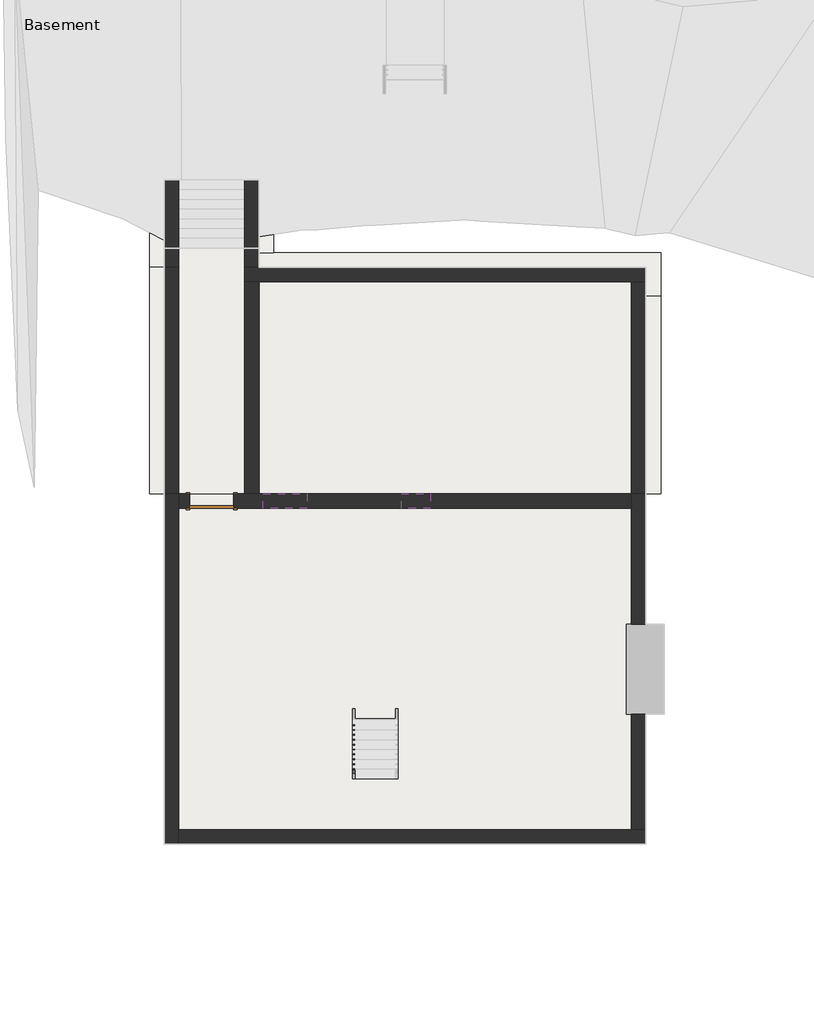
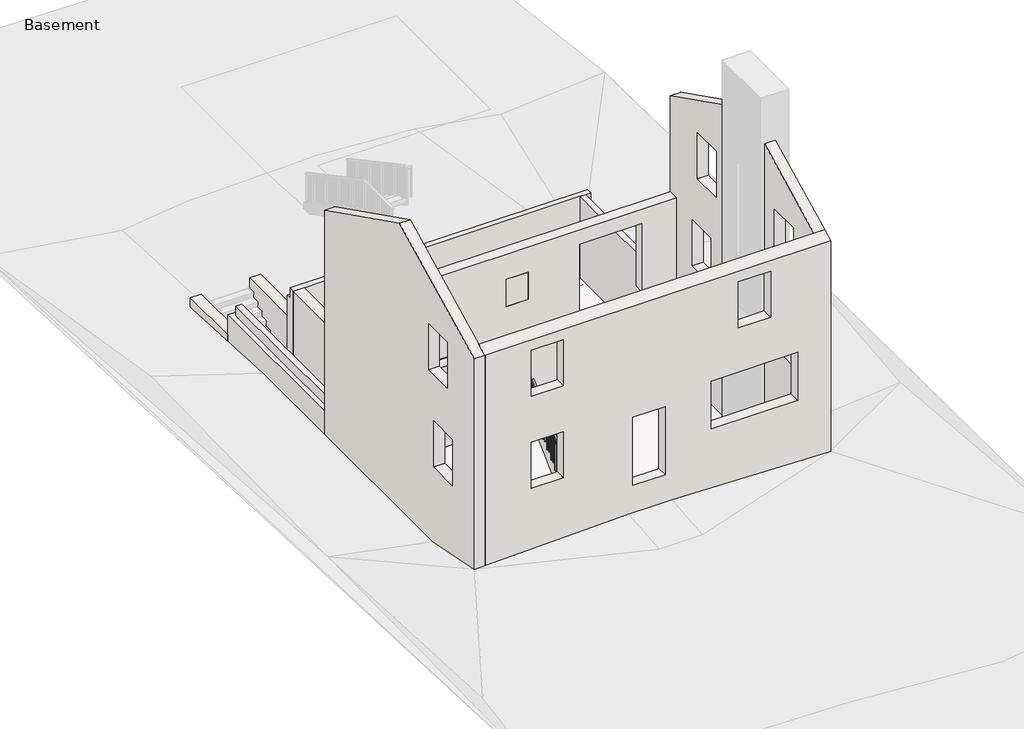
# One storey, part 1 of 3: 13 walls, 6 footings, 4 slabs, 1 door, 1 railing.
"""IFC4 building model written with IfcOpenShell, lengths in millimetres."""

import ifcopenshell
import ifcopenshell.guid

model = None  # the IFC model being written
_history = None  # IfcOwnerHistory: only IFC2X3 demands one
_inside = {}  # id of a spatial element -> (the spatial element, [elements in it])
_under = {}  # id of a project, library or spatial element -> (it, [spatial elements below it])
_declared = {}  # id of a project -> (the project, [libraries it declares])
_typed = {}  # id of a type object -> (the type object, [elements of that type])
_made_of = {}  # id of a material, layer set ... -> (it, [elements and type objects made of it])


def new_model(schema):
    """Start an empty IFC model of exactly this schema.

    Asked for "IFC4X3", IfcOpenShell would pick the latest addendum, in which some entities
    have other attributes; the version numbers below select the first issue.
    IFC2X3 requires an IfcOwnerHistory on every rooted entity: one is made here for all.
    """
    global model, _history
    if schema == "IFC4X3":
        model = ifcopenshell.file(schema_version=(4, 3, 0, 0))
    else:
        model = ifcopenshell.file(schema=schema)
    _inside.clear()
    _under.clear()
    _declared.clear()
    _typed.clear()
    _made_of.clear()
    _history = None
    if model.schema == "IFC2X3":
        org = make("IfcOrganization", Name="unknown")
        user = make(
            "IfcPersonAndOrganization",
            ThePerson=make("IfcPerson", FamilyName="unknown"),
            TheOrganization=org,
        )
        app = make(
            "IfcApplication",
            ApplicationDeveloper=org,
            Version="unknown",
            ApplicationFullName="unknown",
            ApplicationIdentifier="unknown",
        )
        _history = make(
            "IfcOwnerHistory",
            OwningUser=user,
            OwningApplication=app,
            ChangeAction="ADDED",
            CreationDate=0,
        )
    return model


def make(cls, **values):
    """One entity of the class cls with the attributes given. An attribute that is None is left unset."""
    return model.create_entity(
        cls, **{name: value for name, value in values.items() if value is not None}
    )


def rooted(cls, **values):
    """An entity with a GlobalId (a new one), such as an element, a storey or a relation."""
    return make(cls, GlobalId=ifcopenshell.guid.new(), OwnerHistory=_history, **values)


def si_unit(unit_type, name, prefix=None):
    """IfcSIUnit, for example si_unit("LENGTHUNIT", "METRE", prefix="MILLI")."""
    return make("IfcSIUnit", UnitType=unit_type, Prefix=prefix, Name=name)


def assignment(units):
    """IfcUnitAssignment: the units of a project."""
    return None if units is None else make("IfcUnitAssignment", Units=units)


def point(xyz):
    """IfcCartesianPoint."""
    return None if xyz is None else make("IfcCartesianPoint", Coordinates=xyz)


def direction(xyz):
    """IfcDirection."""
    return None if xyz is None else make("IfcDirection", DirectionRatios=xyz)


def frame(location, z_axis=None, x_axis=None):
    """IfcAxis2Placement3D, a coordinate frame: its origin and axes. An axis left out is left unset."""
    return make(
        "IfcAxis2Placement3D",
        Location=point(location),
        Axis=direction(z_axis),
        RefDirection=direction(x_axis),
    )


def origin():
    """The frame at (0, 0, 0) with its axes left unset."""
    return frame((0.0, 0.0, 0.0))


def origin_with_axes():
    """The frame at (0, 0, 0) with the z axis (0, 0, 1) and the x axis (1, 0, 0) written out."""
    return frame((0.0, 0.0, 0.0), z_axis=(0.0, 0.0, 1.0), x_axis=(1.0, 0.0, 0.0))


def place(relative_to, where):
    """IfcLocalPlacement: puts the frame where relative to a parent placement (None: the world)."""
    return make(
        "IfcLocalPlacement", PlacementRelTo=relative_to, RelativePlacement=where
    )


def context(
    kind, dimensions, precision=None, world=None, true_north=None, identifier=None
):
    """IfcGeometricRepresentationContext, for example the 3D "Model" context."""
    return make(
        "IfcGeometricRepresentationContext",
        ContextIdentifier=identifier,
        ContextType=kind,
        CoordinateSpaceDimension=dimensions,
        Precision=precision,
        WorldCoordinateSystem=world,
        TrueNorth=true_north,
    )


def project(units=None, contexts=None):
    """IfcProject with its units and contexts."""
    return rooted(
        "IfcProject",
        Name="project",
        RepresentationContexts=contexts,
        UnitsInContext=assignment(units),
    )


def spatial(cls, under=None, at=None, **own):
    """A site, building, storey or space (cls), placed at a placement, below another one or the project."""
    s = rooted(cls, ObjectPlacement=at, **own)
    if under is not None:
        _under.setdefault(under.id(), (under, []))[1].append(s)
    return s


def polyline(points):
    """IfcPolyline through the points."""
    return make("IfcPolyline", Points=[point(p) for p in points])


def outline(outer, holes=None, kind="AREA"):
    """IfcArbitraryClosedProfileDef: a profile drawn as a closed curve; with holes, ...WithVoids."""
    if holes is None:
        return make("IfcArbitraryClosedProfileDef", ProfileType=kind, OuterCurve=outer)
    return make(
        "IfcArbitraryProfileDefWithVoids",
        ProfileType=kind,
        OuterCurve=outer,
        InnerCurves=holes,
    )


def extrude(swept, where, along, depth):
    """IfcExtrudedAreaSolid: the profile swept, set in the frame where, extruded along a direction by depth."""
    return make(
        "IfcExtrudedAreaSolid",
        SweptArea=swept,
        Position=where,
        ExtrudedDirection=direction(along),
        Depth=depth,
    )


def faces_of(points, faces, orient=None, outer=None):
    """IfcFace entities. A face is a list of loops; a loop is a list of indices into points, from 0.

    orient and outer hold one flag for each loop. By default every Orientation is true, the
    first loop of a face is its IfcFaceOuterBound and the others are IfcFaceBound.
    """
    made = []
    for i, loops in enumerate(faces):
        bounds = []
        for j, loop in enumerate(loops):
            is_outer = j == 0 if outer is None else outer[i][j]
            bounds.append(
                make(
                    "IfcFaceOuterBound" if is_outer else "IfcFaceBound",
                    Bound=make("IfcPolyLoop", Polygon=[points[k] for k in loop]),
                    Orientation=True if orient is None else orient[i][j],
                )
            )
        made.append(make("IfcFace", Bounds=bounds))
    return made


def faceted_brep(points, faces, orient=None, outer=None, voids=None):
    """IfcFacetedBrep: a solid bounded by flat faces; with voids (closed shells), ...WithVoids."""
    shared = [point(p) for p in points]
    hull = make("IfcClosedShell", CfsFaces=faces_of(shared, faces, orient, outer))
    if voids is None:
        return make("IfcFacetedBrep", Outer=hull)
    return make(
        "IfcFacetedBrepWithVoids",
        Outer=hull,
        Voids=[
            make(cls, CfsFaces=faces_of(shared, fs, o, b)) for cls, fs, o, b in voids
        ],
    )


def shape(context_of_items, identifier, shape_type, items):
    """IfcShapeRepresentation: the items that make up one representation, for example the "Body"."""
    return make(
        "IfcShapeRepresentation",
        ContextOfItems=context_of_items,
        RepresentationIdentifier=identifier,
        RepresentationType=shape_type,
        Items=items,
    )


def source(mapping_origin, context_of_items, identifier, shape_type, items):
    """IfcRepresentationMap: a shape defined once, which mapped items show again and again."""
    return make(
        "IfcRepresentationMap",
        MappingOrigin=mapping_origin,
        MappedRepresentation=shape(context_of_items, identifier, shape_type, items),
    )


def transform(
    local_origin,
    x_axis=None,
    y_axis=None,
    z_axis=None,
    scale=None,
    scale2=None,
    scale3=None,
    uniform=True,
):
    """IfcCartesianTransformationOperator3D, or its non-uniform kind. x_axis, y_axis, z_axis: its Axis1, 2, 3."""
    if uniform:
        return make(
            "IfcCartesianTransformationOperator3D",
            Axis1=direction(x_axis),
            Axis2=direction(y_axis),
            LocalOrigin=point(local_origin),
            Scale=scale,
            Axis3=direction(z_axis),
        )
    return make(
        "IfcCartesianTransformationOperator3DnonUniform",
        Axis1=direction(x_axis),
        Axis2=direction(y_axis),
        LocalOrigin=point(local_origin),
        Scale=scale,
        Axis3=direction(z_axis),
        Scale2=scale2,
        Scale3=scale3,
    )


def mapped(mapping_source, mapping_target):
    """IfcMappedItem: shows the shape of a source again, moved by a transform."""
    return make(
        "IfcMappedItem", MappingSource=mapping_source, MappingTarget=mapping_target
    )


def made_of(thing, what):
    """Note that an element or type object is made of a material, layer set ...; save() writes the relation."""
    if what is not None:
        _made_of.setdefault(what.id(), (what, []))[1].append(thing)
    return thing


def element(
    cls,
    number,
    at=None,
    inside=None,
    cuts=None,
    type_object=None,
    material=None,
    context=None,
    identifier="Body",
    shape_type=None,
    held_by="IfcProductDefinitionShape",
    body=None,
    shapes=None,
    **own,
):
    """One element of the class cls, such as IfcWall. Its Tag is "e" and its number.

    at: its placement. inside: the storey or other place that contains it. cuts: it is an
    opening in that element (IfcRelVoidsElement). A single representation is given by context,
    identifier, shape_type and body (its items); several are given by shapes. held_by: the class
    of the entity that holds the representations. save() writes the other relations.
    """
    e = rooted(cls, Tag="e%d" % number, ObjectPlacement=at, **own)
    if body is not None:
        shapes = [shape(context, identifier, shape_type, body)]
    if shapes is not None:
        e.Representation = make(held_by, Representations=shapes)
    if inside is not None:
        _inside.setdefault(inside.id(), (inside, []))[1].append(e)
    if cuts is not None:
        rooted(
            "IfcRelVoidsElement", RelatingBuildingElement=cuts, RelatedOpeningElement=e
        )
    if type_object is not None:
        _typed.setdefault(type_object.id(), (type_object, []))[1].append(e)
    return made_of(e, material)


def aggregate(whole, parts):
    """IfcRelAggregates: a whole, such as a stair, and the parts it consists of."""
    return rooted("IfcRelAggregates", RelatingObject=whole, RelatedObjects=parts)


def save(model, path):
    """Write the relations noted so far, then the file.

    IfcRelAggregates (storeys below a building ...), IfcRelContainedInSpatialStructure (elements
    in a storey), IfcRelDefinesByType, IfcRelAssociatesMaterial and IfcRelDeclares: one each for
    every whole, place, type object, material and project.
    """
    for whole, parts in _under.values():
        aggregate(whole, parts)
    for where, things in _inside.values():
        rooted(
            "IfcRelContainedInSpatialStructure",
            RelatedElements=things,
            RelatingStructure=where,
        )
    for kind, things in _typed.values():
        rooted("IfcRelDefinesByType", RelatedObjects=things, RelatingType=kind)
    for what, things in _made_of.values():
        rooted("IfcRelAssociatesMaterial", RelatedObjects=things, RelatingMaterial=what)
    for by, libraries in _declared.values():
        rooted("IfcRelDeclares", RelatingContext=by, RelatedDefinitions=libraries)
    model.write(path)


def door_03272193(model_context):
    return source(origin(), model_context, "Body", "SweptSolid", [
        extrude(outline(polyline([(2209.8, -533.4), (0.0, -533.4), (0.0, -457.2), (2133.6, -457.2), (2133.6, 457.2), (0.0, 457.2), (0.0, 533.4), (2209.8, 533.4), (2209.8, -533.4)])), frame((0.0, 152.4, 0.0), z_axis=(0.0, 1.0, 0.0), x_axis=(0.0, 0.0, 1.0)), (0.0, 0.0, 1.0), 25.4),
        extrude(outline(polyline([(2209.8, 533.4), (2209.8, -533.4), (0.0, -533.4), (0.0, -457.2), (2133.6, -457.2), (2133.6, 457.2), (0.0, 457.2), (0.0, 533.4), (2209.8, 533.4)])), frame((0.0, -177.8, 0.0), z_axis=(0.0, 1.0, 0.0), x_axis=(0.0, 0.0, 1.0)), (0.0, 0.0, 1.0), 25.4),
        extrude(outline(polyline([(457.2, 101.6), (-457.2, 101.6), (-457.2, 152.4), (457.2, 152.4), (457.2, 101.6)])), origin_with_axes(), (0.0, 0.0, 1.0), 2133.6),
    ])


model = new_model("IFC4")

# Units and contexts
model_context = context("Model", 3, world=origin())
ifc_project = project(units=[si_unit("LENGTHUNIT", "METRE", prefix="MILLI")], contexts=[model_context])

# Site, building, storey
site = spatial("IfcSite", under=ifc_project)
building = spatial("IfcBuilding", under=site)
storey = spatial("IfcBuildingStorey", under=building, Name="Basement", Elevation=-2667.0)

# Door
placement = place(None, origin())
door_shape = door_03272193(model_context)
element("IfcDoor", 1, ObjectType="Single-Flush : 36\" x 84\"", at=placement, inside=storey, context=model_context, shape_type="MappedRepresentation", body=[
    mapped(door_shape, transform((-4998.5803068, 2999.6888758, -2667.0), x_axis=(-1.0, 0.0, 0.0), y_axis=(0.0, -1.0, 0.0), z_axis=(0.0, 0.0, 1.0))),
])

# Footings
element("IfcFooting", 2, ObjectType="Bearing Footing - 36\" x 12\"", at=placement, inside=storey, context=model_context, shape_type="SweptSolid", body=[
    extrude(outline(polyline([(-5379.5803068, 3152.0888758), (-6293.9803068, 3152.0888758), (-6293.9803068, 7876.4888758), (-5379.5803068, 7876.4888758), (-5379.5803068, 3152.0888758)])), frame((0.0, 0.0, -3073.4), z_axis=(0.0, 0.0, 1.0), x_axis=(1.0, 0.0, 0.0)), (0.0, 0.0, 1.0), 304.8),
])
element("IfcFooting", 3, ObjectType="Bearing Footing - 36\" x 12\"", at=placement, inside=storey, context=model_context, shape_type="Brep", body=[
    faceted_brep([(-4160.3803068, 7266.8888758, -2768.6), (-3703.1803068, 7266.8888758, -2768.6), (3459.6196932, 7266.8888758, -2768.6), (4374.0196932, 7266.8888758, -2768.6), (4374.0196932, 8181.2888758, -2768.6), (-3703.1803068, 8181.2888758, -2768.6), (-4160.3803068, 8181.2888758, -2768.6), (-4160.3803068, 7876.4888758, -2768.6), (-4160.3803068, 7724.0888758, -2768.6), (-4160.3803068, 7571.6888758, -2768.6), (-4160.3803068, 8181.2888758, -3073.4), (4374.0196932, 8181.2888758, -3073.4), (-3703.1803068, 8181.2888758, -3073.4), (-4160.3803068, 7266.8888758, -3073.4), (-4160.3803068, 7571.6888758, -3073.4), (-4160.3803068, 7724.0888758, -3073.4), (-4160.3803068, 7876.4888758, -3073.4), (4374.0196932, 7266.8888758, -3073.4), (3459.6196932, 7266.8888758, -3073.4), (-3703.1803068, 7266.8888758, -3073.4)], [[[0, 1, 2, 3, 4, 5, 6, 7, 8, 9]], [[10, 6, 5, 4, 11, 12]], [[13, 14, 15, 16, 10, 12, 11, 17, 18, 19]], [[0, 13, 19, 18, 17, 3, 2, 1]], [[4, 3, 17, 11]], [[0, 9, 8, 15, 14, 13]], [[8, 7, 6, 10, 16, 15]]]),
])
element("IfcFooting", 4, ObjectType="Bearing Footing - 36\" x 12\"", at=placement, inside=storey, context=model_context, shape_type="SweptSolid", body=[
    extrude(outline(polyline([(4374.0196932, 3152.0888758), (3459.6196932, 3152.0888758), (3459.6196932, 7266.8888758), (4374.0196932, 7266.8888758), (4374.0196932, 3152.0888758)])), frame((0.0, 0.0, -3073.4), z_axis=(0.0, 0.0, 1.0), x_axis=(1.0, 0.0, 0.0)), (0.0, 0.0, 1.0), 304.8),
])
element("IfcFooting", 5, ObjectType="Bearing Footing - 36\" x 12\"", at=placement, inside=storey, context=model_context, shape_type="SweptSolid", body=[
    extrude(outline(polyline([(-3703.1803068, 3152.0888758), (-4617.5803068, 3152.0888758), (-4617.5803068, 7571.6888758), (-4160.3803068, 7571.6888758), (-4160.3803068, 7266.8888758), (-3703.1803068, 7266.8888758), (-3703.1803068, 3152.0888758)])), frame((0.0, 0.0, -3073.4), z_axis=(0.0, 0.0, 1.0), x_axis=(1.0, 0.0, 0.0)), (0.0, 0.0, 1.0), 304.8),
])
element("IfcFooting", 6, ObjectType="Bearing Footing - 36\" x 12\"", at=placement, inside=storey, context=model_context, shape_type="SweptSolid", body=[
    extrude(outline(polyline([(-4617.5803068, 9705.2888758), (-3703.1803068, 9705.2888758), (-3703.1803068, 8181.2888758), (-4160.3803068, 8181.2888758), (-4160.3803068, 7876.4888758), (-4617.5803068, 7876.4888758), (-4617.5803068, 9705.2888758)])), frame((0.0, 0.0, -3073.4), z_axis=(0.0, 0.0, 1.0), x_axis=(1.0, 0.0, 0.0)), (0.0, 0.0, 1.0), 304.8),
])
element("IfcFooting", 7, ObjectType="Bearing Footing - 36\" x 12\"", at=placement, inside=storey, context=model_context, shape_type="SweptSolid", body=[
    extrude(outline(polyline([(-5379.5803068, 7876.4888758), (-6293.9803068, 7876.4888758), (-6293.9803068, 9705.2888758), (-5379.5803068, 9705.2888758), (-5379.5803068, 7876.4888758)])), frame((0.0, 0.0, -3073.4), z_axis=(0.0, 0.0, 1.0), x_axis=(1.0, 0.0, 0.0)), (0.0, 0.0, 1.0), 304.8),
])

# Railing
element("IfcRailing", 8, ObjectType="Handrail - Rectangular", at=placement, inside=storey, context=model_context, shape_type="SweptSolid", body=[
    extrude(outline(polyline([(-2791.5111242, -1631.7331862), (-2791.5111242, -1562.1), (-149.9111242, 914.4), (-149.9111242, 844.7668138), (-2791.5111242, -1631.7331862)])), frame((-2052.1803068, 0.0, 0.0), z_axis=(1.0, 0.0, 0.0), x_axis=(0.0, 1.0, 0.0)), (0.0, 0.0, 1.0), 50.8),
    extrude(outline(polyline([(-241.9861242, 758.4465013), (-241.9861242, -190.5), (-261.0361242, -190.5), (-261.0361242, 740.5871263), (-241.9861242, 758.4465013)])), frame((-2036.3053068, 0.0, 0.0), z_axis=(1.0, 0.0, 0.0), x_axis=(0.0, 1.0, 0.0)), (0.0, 0.0, 1.0), 19.05),
    extrude(outline(polyline([(-343.5861242, 663.1965013), (-343.5861242, -190.5), (-362.6361242, -190.5), (-362.6361242, 645.3371263), (-343.5861242, 663.1965013)])), frame((-2036.3053068, 0.0, 0.0), z_axis=(1.0, 0.0, 0.0), x_axis=(0.0, 1.0, 0.0)), (0.0, 0.0, 1.0), 19.05),
    extrude(outline(polyline([(-445.1861242, 567.9465013), (-445.1861242, -381.0), (-464.2361242, -381.0), (-464.2361242, 550.0871263), (-445.1861242, 567.9465013)])), frame((-2036.3053068, 0.0, 0.0), z_axis=(1.0, 0.0, 0.0), x_axis=(0.0, 1.0, 0.0)), (0.0, 0.0, 1.0), 19.05),
    extrude(outline(polyline([(-546.7861242, 472.6965013), (-546.7861242, -381.0), (-565.8361242, -381.0), (-565.8361242, 454.8371263), (-546.7861242, 472.6965013)])), frame((-2036.3053068, 0.0, 0.0), z_axis=(1.0, 0.0, 0.0), x_axis=(0.0, 1.0, 0.0)), (0.0, 0.0, 1.0), 19.05),
    extrude(outline(polyline([(-648.3861242, 377.4465013), (-648.3861242, -571.5), (-667.4361242, -571.5), (-667.4361242, 359.5871263), (-648.3861242, 377.4465013)])), frame((-2036.3053068, 0.0, 0.0), z_axis=(1.0, 0.0, 0.0), x_axis=(0.0, 1.0, 0.0)), (0.0, 0.0, 1.0), 19.05),
    extrude(outline(polyline([(-749.9861242, 282.1965013), (-749.9861242, -571.5), (-769.0361242, -571.5), (-769.0361242, 264.3371263), (-749.9861242, 282.1965013)])), frame((-2036.3053068, 0.0, 0.0), z_axis=(1.0, 0.0, 0.0), x_axis=(0.0, 1.0, 0.0)), (0.0, 0.0, 1.0), 19.05),
    extrude(outline(polyline([(-851.5861242, 186.9465013), (-851.5861242, -762.0), (-870.6361242, -762.0), (-870.6361242, 169.0871263), (-851.5861242, 186.9465013)])), frame((-2036.3053068, 0.0, 0.0), z_axis=(1.0, 0.0, 0.0), x_axis=(0.0, 1.0, 0.0)), (0.0, 0.0, 1.0), 19.05),
    extrude(outline(polyline([(-953.1861242, 91.6965013), (-953.1861242, -762.0), (-972.2361242, -762.0), (-972.2361242, 73.8371263), (-953.1861242, 91.6965013)])), frame((-2036.3053068, 0.0, 0.0), z_axis=(1.0, 0.0, 0.0), x_axis=(0.0, 1.0, 0.0)), (0.0, 0.0, 1.0), 19.05),
    extrude(outline(polyline([(-1054.7861242, -3.5534987), (-1054.7861242, -952.5), (-1073.8361242, -952.5), (-1073.8361242, -21.4128737), (-1054.7861242, -3.5534987)])), frame((-2036.3053068, 0.0, 0.0), z_axis=(1.0, 0.0, 0.0), x_axis=(0.0, 1.0, 0.0)), (0.0, 0.0, 1.0), 19.05),
    extrude(outline(polyline([(-1156.3861242, -98.8034987), (-1156.3861242, -952.5), (-1175.4361242, -952.5), (-1175.4361242, -116.6628737), (-1156.3861242, -98.8034987)])), frame((-2036.3053068, 0.0, 0.0), z_axis=(1.0, 0.0, 0.0), x_axis=(0.0, 1.0, 0.0)), (0.0, 0.0, 1.0), 19.05),
    extrude(outline(polyline([(-1257.9861242, -194.0534987), (-1257.9861242, -1143.0), (-1277.0361242, -1143.0), (-1277.0361242, -211.9128737), (-1257.9861242, -194.0534987)])), frame((-2036.3053068, 0.0, 0.0), z_axis=(1.0, 0.0, 0.0), x_axis=(0.0, 1.0, 0.0)), (0.0, 0.0, 1.0), 19.05),
    extrude(outline(polyline([(-1359.5861242, -289.3034987), (-1359.5861242, -1143.0), (-1378.6361242, -1143.0), (-1378.6361242, -307.1628737), (-1359.5861242, -289.3034987)])), frame((-2036.3053068, 0.0, 0.0), z_axis=(1.0, 0.0, 0.0), x_axis=(0.0, 1.0, 0.0)), (0.0, 0.0, 1.0), 19.05),
    extrude(outline(polyline([(-1461.1861242, -384.5534987), (-1461.1861242, -1333.5), (-1480.2361242, -1333.5), (-1480.2361242, -402.4128737), (-1461.1861242, -384.5534987)])), frame((-2036.3053068, 0.0, 0.0), z_axis=(1.0, 0.0, 0.0), x_axis=(0.0, 1.0, 0.0)), (0.0, 0.0, 1.0), 19.05),
    extrude(outline(polyline([(-1562.7861242, -479.8034987), (-1562.7861242, -1333.5), (-1581.8361242, -1333.5), (-1581.8361242, -497.6628737), (-1562.7861242, -479.8034987)])), frame((-2036.3053068, 0.0, 0.0), z_axis=(1.0, 0.0, 0.0), x_axis=(0.0, 1.0, 0.0)), (0.0, 0.0, 1.0), 19.05),
    extrude(outline(polyline([(-1664.3861242, -575.0534987), (-1664.3861242, -1524.0), (-1683.4361242, -1524.0), (-1683.4361242, -592.9128737), (-1664.3861242, -575.0534987)])), frame((-2036.3053068, 0.0, 0.0), z_axis=(1.0, 0.0, 0.0), x_axis=(0.0, 1.0, 0.0)), (0.0, 0.0, 1.0), 19.05),
    extrude(outline(polyline([(-1765.9861242, -670.3034987), (-1765.9861242, -1524.0), (-1785.0361242, -1524.0), (-1785.0361242, -688.1628737), (-1765.9861242, -670.3034987)])), frame((-2036.3053068, 0.0, 0.0), z_axis=(1.0, 0.0, 0.0), x_axis=(0.0, 1.0, 0.0)), (0.0, 0.0, 1.0), 19.05),
    extrude(outline(polyline([(-1867.5861242, -765.5534987), (-1867.5861242, -1714.5), (-1886.6361242, -1714.5), (-1886.6361242, -783.4128737), (-1867.5861242, -765.5534987)])), frame((-2036.3053068, 0.0, 0.0), z_axis=(1.0, 0.0, 0.0), x_axis=(0.0, 1.0, 0.0)), (0.0, 0.0, 1.0), 19.05),
    extrude(outline(polyline([(-1969.1861242, -860.8034987), (-1969.1861242, -1714.5), (-1988.2361242, -1714.5), (-1988.2361242, -878.6628737), (-1969.1861242, -860.8034987)])), frame((-2036.3053068, 0.0, 0.0), z_axis=(1.0, 0.0, 0.0), x_axis=(0.0, 1.0, 0.0)), (0.0, 0.0, 1.0), 19.05),
    extrude(outline(polyline([(-2070.7861242, -956.0534987), (-2070.7861242, -1905.0), (-2089.8361242, -1905.0), (-2089.8361242, -973.9128737), (-2070.7861242, -956.0534987)])), frame((-2036.3053068, 0.0, 0.0), z_axis=(1.0, 0.0, 0.0), x_axis=(0.0, 1.0, 0.0)), (0.0, 0.0, 1.0), 19.05),
    extrude(outline(polyline([(-2172.3861242, -1051.3034987), (-2172.3861242, -1905.0), (-2191.4361242, -1905.0), (-2191.4361242, -1069.1628737), (-2172.3861242, -1051.3034987)])), frame((-2036.3053068, 0.0, 0.0), z_axis=(1.0, 0.0, 0.0), x_axis=(0.0, 1.0, 0.0)), (0.0, 0.0, 1.0), 19.05),
    extrude(outline(polyline([(-2273.9861242, -1146.5534987), (-2273.9861242, -2095.5), (-2293.0361242, -2095.5), (-2293.0361242, -1164.4128737), (-2273.9861242, -1146.5534987)])), frame((-2036.3053068, 0.0, 0.0), z_axis=(1.0, 0.0, 0.0), x_axis=(0.0, 1.0, 0.0)), (0.0, 0.0, 1.0), 19.05),
    extrude(outline(polyline([(-2375.5861242, -1241.8034987), (-2375.5861242, -2095.5), (-2394.6361242, -2095.5), (-2394.6361242, -1259.6628737), (-2375.5861242, -1241.8034987)])), frame((-2036.3053068, 0.0, 0.0), z_axis=(1.0, 0.0, 0.0), x_axis=(0.0, 1.0, 0.0)), (0.0, 0.0, 1.0), 19.05),
    extrude(outline(polyline([(-2477.1861242, -1337.0534987), (-2477.1861242, -2286.0), (-2496.2361242, -2286.0), (-2496.2361242, -1354.9128737), (-2477.1861242, -1337.0534987)])), frame((-2036.3053068, 0.0, 0.0), z_axis=(1.0, 0.0, 0.0), x_axis=(0.0, 1.0, 0.0)), (0.0, 0.0, 1.0), 19.05),
    extrude(outline(polyline([(-2578.7861242, -1432.3034987), (-2578.7861242, -2286.0), (-2597.8361242, -2286.0), (-2597.8361242, -1450.1628737), (-2578.7861242, -1432.3034987)])), frame((-2036.3053068, 0.0, 0.0), z_axis=(1.0, 0.0, 0.0), x_axis=(0.0, 1.0, 0.0)), (0.0, 0.0, 1.0), 19.05),
    extrude(outline(polyline([(-2680.3861242, -1527.5534987), (-2680.3861242, -2476.5), (-2699.4361242, -2476.5), (-2699.4361242, -1545.4128737), (-2680.3861242, -1527.5534987)])), frame((-2036.3053068, 0.0, 0.0), z_axis=(1.0, 0.0, 0.0), x_axis=(0.0, 1.0, 0.0)), (0.0, 0.0, 1.0), 19.05),
    extrude(outline(polyline([(-149.9111242, 844.7668138), (-149.9111242, -190.5), (-168.9611242, -190.5), (-168.9611242, 826.9074388), (-149.9111242, 844.7668138)])), frame((-2036.3053068, 0.0, 0.0), z_axis=(1.0, 0.0, 0.0), x_axis=(0.0, 1.0, 0.0)), (0.0, 0.0, 1.0), 19.05),
    extrude(outline(polyline([(-2772.4611242, -1613.8738112), (-2772.4611242, -2476.5), (-2791.5111242, -2476.5), (-2791.5111242, -1631.7331862), (-2772.4611242, -1613.8738112)])), frame((-2036.3053068, 0.0, 0.0), z_axis=(1.0, 0.0, 0.0), x_axis=(0.0, 1.0, 0.0)), (0.0, 0.0, 1.0), 19.05),
])

# Slabs
element("IfcSlab", 9, ObjectType="4\" Concrete", at=placement, inside=storey, context=model_context, shape_type="Brep", body=[
    faceted_brep([(-5684.3803068, 8384.4888758, -2768.6), (-4312.7803068, 8384.4888758, -2768.6), (-4312.7803068, 7876.4888758, -2768.6), (-4312.7803068, 7571.6888758, -2768.6), (-4312.7803068, 3152.0888758, -2768.6), (-5684.3803068, 3152.0888758, -2768.6), (-5684.3803068, 7876.4888758, -2768.6), (-5684.3803068, 8384.4888758, -2667.0), (-5684.3803068, 3152.0888758, -2667.0), (-4312.7803068, 3152.0888758, -2667.0), (-4312.7803068, 8384.4888758, -2667.0)], [[[0, 1, 2, 3, 4, 5, 6]], [[7, 8, 9, 10]], [[1, 0, 7, 10]], [[4, 3, 2, 1, 10, 9]], [[5, 4, 9, 8]], [[0, 6, 5, 8, 7]]]),
])
element("IfcSlab", 10, ObjectType="Pad 1", at=placement, inside=storey, context=model_context, shape_type="SweptSolid", body=[
    extrude(outline(polyline([(4069.2196932, 434.2888758), (4450.2196932, 434.2888758), (4450.2196932, -1445.3111242), (4069.2196932, -1445.3111242), (4069.2196932, -4163.1111242), (-5989.1803068, -4163.1111242), (-5989.1803068, 3152.0888758), (4069.2196932, 3152.0888758), (4069.2196932, 434.2888758)])), frame((0.0, 0.0, -2774.95), z_axis=(0.0, 0.0, 1.0), x_axis=(1.0, 0.0, 0.0)), (0.0, 0.0, 1.0), 6.35),
])
element("IfcSlab", 11, ObjectType="Pad 1", at=placement, inside=storey, context=model_context, shape_type="SweptSolid", body=[
    extrude(outline(polyline([(-5989.1803068, 8275.4102719), (-4007.9803068, 8275.4102719), (-4007.9803068, 7876.4888758), (4069.2196932, 7876.4888758), (4069.2196932, 3152.0888758), (-5989.1803068, 3152.0888758), (-5989.1803068, 8275.4102719)])), frame((0.0, 0.0, -2774.95), z_axis=(0.0, 0.0, 1.0), x_axis=(1.0, 0.0, 0.0)), (0.0, 0.0, 1.0), 6.35),
])
element("IfcSlab", 12, ObjectType="Pad 1", at=placement, inside=storey, context=model_context, shape_type="SweptSolid", body=[
    extrude(outline(polyline([(9705.2888758, -1653.200634), (8275.4102719, -2776.6756068), (8275.4102719, -2768.6), (9705.2888758, -1645.1250272), (9705.2888758, -1653.200634)])), frame((-5989.1803068, 0.0, 0.0), z_axis=(1.0, 0.0, 0.0), x_axis=(0.0, 1.0, 0.0)), (0.0, 0.0, 1.0), 1981.2),
])

# Walls
element("IfcWall", 13, ObjectType="Foundation - 12\" Concrete", at=placement, inside=storey, context=model_context, shape_type="Brep", body=[
    faceted_brep([(-5684.3803068, 3152.0888758, -2768.6), (-5684.3803068, 7876.4888758, -2768.6), (-5684.3803068, 7876.4888758, -1244.6), (-5684.3803068, 7876.4888758, -654.05), (-5684.3803068, 7733.6138758, -654.05), (-5684.3803068, 7733.6138758, -349.25), (-5684.3803068, 3152.0888758, -349.25), (-5684.3803068, 3152.0888758, -2667.0), (-5989.1803068, 7876.4888758, -2768.6), (-5989.1803068, 3152.0888758, -2768.6), (-5989.1803068, 3152.0888758, -654.05), (-5989.1803068, 7876.4888758, -654.05), (-5989.1803068, 7876.4888758, -1244.6), (-5846.3053068, 3152.0888758, -349.25), (-5846.3053068, 3152.0888758, -654.05), (-5846.3053068, 7876.4888758, -654.05), (-5846.3053068, 7733.6138758, -349.25), (-5846.3053068, 7733.6138758, -654.05)], [[[0, 1, 2, 3, 4, 5, 6, 7]], [[8, 9, 10, 11, 12]], [[0, 7, 6, 13, 14, 10, 9]], [[1, 0, 9, 8]], [[1, 8, 12, 11, 15, 3, 2]], [[13, 6, 5, 16]], [[14, 13, 16, 17]], [[11, 10, 14, 17, 4, 3, 15]], [[4, 17, 16, 5]]]),
])
element("IfcWall", 14, ObjectType="Foundation - 12\" Concrete", at=placement, inside=storey, context=model_context, shape_type="Brep", body=[
    faceted_brep([(-4312.7803068, 7571.6888758, -2768.6), (-4007.9803068, 7571.6888758, -2768.6), (3764.4196932, 7571.6888758, -2768.6), (4069.2196932, 7571.6888758, -2768.6), (4069.2196932, 7571.6888758, -654.05), (4069.2196932, 7571.6888758, -349.25), (3926.3446932, 7571.6888758, -349.25), (3764.4196932, 7571.6888758, -349.25), (-4007.9803068, 7571.6888758, -349.25), (-4312.7803068, 7571.6888758, -349.25), (4069.2196932, 7876.4888758, -2768.6), (-4007.9803068, 7876.4888758, -2768.6), (-4312.7803068, 7876.4888758, -2768.6), (-4312.7803068, 7876.4888758, -1244.6), (-4312.7803068, 7876.4888758, -654.05), (4069.2196932, 7876.4888758, -654.05), (4069.2196932, 7733.6138758, -654.05), (4069.2196932, 7733.6138758, -349.25), (-4312.7803068, 7733.6138758, -349.25), (-4312.7803068, 7733.6138758, -654.05)], [[[0, 1, 2, 3, 4, 5, 6, 7, 8, 9]], [[10, 11, 12, 13, 14, 15]], [[5, 4, 3, 10, 15, 16, 17]], [[3, 2, 1, 0, 12, 11, 10]], [[9, 8, 7, 6, 5, 17, 18]], [[12, 0, 9, 18, 19, 14, 13]], [[16, 19, 18, 17]], [[19, 16, 15, 14]]]),
])
element("IfcWall", 15, ObjectType="Foundation - 12\" Concrete", at=placement, inside=storey, context=model_context, shape_type="Brep", body=[
    faceted_brep([(3764.4196932, 7571.6888758, -2768.6), (3764.4196932, 3152.0888758, -2768.6), (3764.4196932, 3152.0888758, -349.25), (3764.4196932, 7558.9888758, -349.25), (3764.4196932, 7571.6888758, -349.25), (4069.2196932, 3152.0888758, -2768.6), (4069.2196932, 7571.6888758, -2768.6), (4069.2196932, 7571.6888758, -654.05), (4069.2196932, 3152.0888758, -654.05), (3926.3446932, 3152.0888758, -349.25), (3926.3446932, 7558.9888758, -349.25), (3926.3446932, 7571.6888758, -349.25), (3926.3446932, 3152.0888758, -654.05), (3926.3446932, 7571.6888758, -654.05)], [[[0, 1, 2, 3, 4]], [[5, 6, 7, 8]], [[1, 0, 6, 5]], [[3, 2, 9, 10, 11, 4]], [[2, 1, 5, 8, 12, 9]], [[0, 4, 11, 13, 7, 6]], [[12, 13, 11, 10, 9]], [[13, 12, 8, 7]]]),
])
element("IfcWall", 16, ObjectType="Foundation - 12\" Concrete", at=placement, inside=storey, context=model_context, shape_type="Brep", body=[
    faceted_brep([(-4007.9803068, 3152.0888758, -2768.6), (-4007.9803068, 7571.6888758, -2768.6), (-4007.9803068, 7571.6888758, -349.25), (-4007.9803068, 3152.0888758, -349.25), (-4312.7803068, 3152.0888758, -2768.6), (-4312.7803068, 3152.0888758, -2667.0), (-4312.7803068, 3152.0888758, -349.25), (-4312.7803068, 7571.6888758, -349.25), (-4312.7803068, 7571.6888758, -2768.6)], [[[0, 1, 2, 3]], [[4, 5, 6, 7, 8]], [[0, 3, 6, 5, 4]], [[1, 0, 4, 8]], [[3, 2, 7, 6]], [[1, 8, 7, 2]]]),
])
element("IfcWall", 17, ObjectType="Foundation - 12\" Concrete", at=placement, inside=storey, context=model_context, shape_type="Brep", body=[
    faceted_brep([(-4007.9803068, 7876.4888758, -2768.6), (-4007.9803068, 9705.2888758, -2768.6), (-4007.9803068, 9705.2888758, -1244.6), (-4007.9803068, 7876.4888758, -1244.6), (-4312.7803068, 7876.4888758, -2768.6), (-4312.7803068, 7876.4888758, -1244.6), (-4312.7803068, 9705.2888758, -1244.6), (-4312.7803068, 9705.2888758, -2768.6), (-4312.7803068, 8384.4888758, -2768.6)], [[[0, 1, 2, 3]], [[4, 5, 6, 7, 8]], [[1, 0, 4, 8, 7]], [[2, 1, 7, 6]], [[3, 2, 6, 5]], [[0, 3, 5, 4]]]),
])
element("IfcWall", 18, ObjectType="Foundation - 12\" Concrete", at=placement, inside=storey, context=model_context, shape_type="Brep", body=[
    faceted_brep([(-5684.3803068, 7876.4888758, -2768.6), (-5684.3803068, 8384.4888758, -2768.6), (-5684.3803068, 9705.2888758, -2768.6), (-5684.3803068, 9705.2888758, -1244.6), (-5684.3803068, 7876.4888758, -1244.6), (-5989.1803068, 7876.4888758, -2768.6), (-5989.1803068, 7876.4888758, -1244.6), (-5989.1803068, 9705.2888758, -1244.6), (-5989.1803068, 9705.2888758, -2768.6)], [[[0, 1, 2, 3, 4]], [[5, 6, 7, 8]], [[2, 1, 0, 5, 8]], [[3, 2, 8, 7]], [[4, 3, 7, 6]], [[0, 4, 6, 5]]]),
])
element("IfcWall", 19, ObjectType="Generic - 12\"", at=placement, inside=storey, context=model_context, shape_type="Brep", body=[
    faceted_brep([(1021.2196932, 2847.2888758, 0.0), (1021.2196932, 2847.2888758, 2057.4), (2799.2196932, 2847.2888758, 2057.4), (2799.2196932, 2847.2888758, 0.0), (3764.4196932, 2847.2888758, 0.0), (3764.4196932, 2847.2888758, 2470.15), (-680.5803068, 2847.2888758, 2470.15), (-5684.3803068, 2847.2888758, 2470.15), (-5684.3803068, 2847.2888758, 0.0), (-5023.9803068, 2847.2888758, 0.0), (-5023.9803068, 2847.2888758, 2032.0), (-4160.3803068, 2847.2888758, 2032.0), (-4160.3803068, 2847.2888758, 0.0), (-1518.7803068, 2847.2888758, 0.0), (-1391.7803068, 2847.2888758, 0.0), (-70.9803068, 2847.2888758, 0.0), (56.0196932, 2847.2888758, 0.0), (-3919.0803068, 2847.2888758, 914.4), (-3919.0803068, 2847.2888758, 1727.2), (-3004.6803068, 2847.2888758, 1727.2), (-3004.6803068, 2847.2888758, 914.4), (-1036.1803068, 2847.2888758, 914.4), (-1036.1803068, 2847.2888758, 1727.2), (-426.5803068, 2847.2888758, 1727.2), (-426.5803068, 2847.2888758, 914.4), (1021.2196932, 3152.0888758, 2057.4), (1021.2196932, 3152.0888758, 0.0), (-4160.3803068, 3152.0888758, 0.0), (-4160.3803068, 3152.0888758, 2032.0), (-5023.9803068, 3152.0888758, 2032.0), (-5023.9803068, 3152.0888758, 0.0), (-5684.3803068, 3152.0888758, 0.0), (-5684.3803068, 3152.0888758, 2470.15), (3764.4196932, 3152.0888758, 2470.15), (3764.4196932, 3152.0888758, 0.0), (2799.2196932, 3152.0888758, 0.0), (2799.2196932, 3152.0888758, 2057.4), (-3919.0803068, 3152.0888758, 1727.2), (-3919.0803068, 3152.0888758, 914.4), (-3004.6803068, 3152.0888758, 914.4), (-3004.6803068, 3152.0888758, 1727.2), (-1036.1803068, 3152.0888758, 1727.2), (-1036.1803068, 3152.0888758, 914.4), (-426.5803068, 3152.0888758, 914.4), (-426.5803068, 3152.0888758, 1727.2)], [[[0, 1, 2, 3, 4, 5, 6, 7, 8, 9, 10, 11, 12, 13, 14, 15, 16], [17, 18, 19, 20], [21, 22, 23, 24]], [[25, 26, 27, 28, 29, 30, 31, 32, 33, 34, 35, 36], [37, 38, 39, 40], [41, 42, 43, 44]], [[25, 1, 0, 26]], [[1, 25, 36, 2]], [[2, 36, 35, 3]], [[10, 9, 30, 29]], [[11, 10, 29, 28]], [[12, 11, 28, 27]], [[9, 8, 31, 30]], [[4, 3, 35, 34]], [[0, 16, 15, 14, 13, 12, 27, 26]], [[7, 6, 5, 33, 32]], [[4, 34, 33, 5]], [[37, 18, 17, 38]], [[38, 17, 20, 39]], [[39, 20, 19, 40]], [[18, 37, 40, 19]], [[41, 22, 21, 42]], [[42, 21, 24, 43]], [[43, 24, 23, 44]], [[22, 41, 44, 23]], [[31, 8, 7, 32]]]),
    faceted_brep([(3764.4196932, 2847.2888758, -273.05), (-5684.3803068, 2847.2888758, -273.05), (-5684.3803068, 2847.2888758, -2667.0), (-5455.7803068, 2847.2888758, -2667.0), (-5455.7803068, 2847.2888758, -533.4), (-4541.3803068, 2847.2888758, -533.4), (-4541.3803068, 2847.2888758, -2667.0), (3764.4196932, 2847.2888758, -2667.0), (-5684.3803068, 3152.0888758, -273.05), (3764.4196932, 3152.0888758, -273.05), (3764.4196932, 3152.0888758, -2667.0), (-4541.3803068, 3152.0888758, -2667.0), (-4541.3803068, 3152.0888758, -533.4), (-5455.7803068, 3152.0888758, -533.4), (-5455.7803068, 3152.0888758, -2667.0), (-5684.3803068, 3152.0888758, -2667.0)], [[[0, 1, 2, 3, 4, 5, 6, 7]], [[8, 9, 10, 11, 12, 13, 14, 15]], [[10, 7, 6, 11]], [[3, 2, 15, 14]], [[1, 0, 9, 8]], [[7, 10, 9, 0]], [[13, 4, 3, 14]], [[4, 13, 12, 5]], [[5, 12, 11, 6]], [[15, 2, 1, 8]]]),
])
element("IfcWall", 20, ObjectType="Generic - 12\"", at=placement, inside=storey, context=model_context, shape_type="Brep", body=[
    faceted_brep([(-5684.3803068, -4163.1111242, -2667.0), (-5684.3803068, -3858.3111242, -2667.0), (-5684.3803068, 2847.2888758, -2667.0), (-5684.3803068, 3152.0888758, -2667.0), (-5684.3803068, 3152.0888758, -273.05), (-5684.3803068, 3152.0888758, 0.0), (-5684.3803068, 3152.0888758, 2470.15), (-5684.3803068, 2847.2888758, 2470.15), (-5684.3803068, 1450.2888758, 2470.15), (-5684.3803068, 1450.2888758, 2743.2), (-5684.3803068, 3152.0888758, 2743.2), (-5684.3803068, 3152.0888758, 5336.1342644), (-5684.3803068, 3147.820347, 5336.1342644), (-5684.3803068, -505.5111242, 7162.8), (-5684.3803068, -3858.3111242, 5486.4), (-5684.3803068, -4158.8425953, 5336.1342644), (-5684.3803068, -4163.1111242, 5336.1342644), (-5684.3803068, -3096.3111242, 914.4), (-5684.3803068, -3096.3111242, 2286.0), (-5684.3803068, -2181.9111242, 2286.0), (-5684.3803068, -2181.9111242, 914.4), (-5684.3803068, -2842.3111242, 3657.6), (-5684.3803068, -2842.3111242, 5029.2), (-5684.3803068, -1927.9111242, 5029.2), (-5684.3803068, -1927.9111242, 3657.6), (-5989.1803068, 3152.0888758, -2667.0), (-5989.1803068, -4163.1111242, -2667.0), (-5989.1803068, -4163.1111242, 5336.1342644), (-5989.1803068, -4158.8425953, 5336.1342644), (-5989.1803068, -505.5111242, 7162.8), (-5989.1803068, 3147.820347, 5336.1342644), (-5989.1803068, 3152.0888758, 5336.1342644), (-5989.1803068, -3096.3111242, 2286.0), (-5989.1803068, -3096.3111242, 914.4), (-5989.1803068, -2181.9111242, 914.4), (-5989.1803068, -2181.9111242, 2286.0), (-5989.1803068, -2842.3111242, 5029.2), (-5989.1803068, -2842.3111242, 3657.6), (-5989.1803068, -1927.9111242, 3657.6), (-5989.1803068, -1927.9111242, 5029.2), (-5827.2553068, 3152.0888758, 2743.2), (-5827.2553068, 3152.0888758, 2470.15), (-5827.2553068, 1450.2888758, 2470.15), (-5827.2553068, 1450.2888758, 2743.2)], [[[0, 1, 2, 3, 4, 5, 6, 7, 8, 9, 10, 11, 12, 13, 14, 15, 16], [17, 18, 19, 20], [21, 22, 23, 24]], [[25, 26, 27, 28, 29, 30, 31], [32, 33, 34, 35], [36, 37, 38, 39]], [[3, 2, 1, 0, 26, 25]], [[0, 16, 27, 26]], [[33, 32, 18, 17]], [[34, 33, 17, 20]], [[35, 34, 20, 19]], [[32, 35, 19, 18]], [[22, 21, 37, 36]], [[21, 24, 38, 37]], [[24, 23, 39, 38]], [[23, 22, 36, 39]], [[27, 16, 15, 28]], [[29, 28, 15, 14, 13]], [[13, 12, 30, 29]], [[12, 11, 31, 30]], [[3, 25, 31, 11, 10, 40, 41, 6, 5, 4]], [[41, 42, 8, 7, 6]], [[9, 43, 40, 10]], [[43, 42, 41, 40]], [[42, 43, 9, 8]]]),
])
element("IfcWall", 21, ObjectType="Generic - 12\"", at=placement, inside=storey, context=model_context, shape_type="Brep", body=[
    faceted_brep([(4069.2196932, -3858.3111242, -2667.0), (3764.4196932, -3858.3111242, -2667.0), (-5684.3803068, -3858.3111242, -2667.0), (-5684.3803068, -3858.3111242, 5486.4), (3764.4196932, -3858.3111242, 5486.4), (4069.2196932, -3858.3111242, 5486.4), (-1518.7803068, -3858.3111242, 0.0), (-604.3803068, -3858.3111242, 0.0), (-604.3803068, -3858.3111242, 2032.0), (-1518.7803068, -3858.3111242, 2032.0), (-3474.5803068, -3858.3111242, 2286.0), (-4388.9803068, -3858.3111242, 2286.0), (-4388.9803068, -3858.3111242, 914.4), (-3474.5803068, -3858.3111242, 914.4), (691.0196932, -3858.3111242, 2336.8), (691.0196932, -3858.3111242, 914.4), (3129.4196932, -3858.3111242, 914.4), (3129.4196932, -3858.3111242, 2336.8), (2367.4196932, -3858.3111242, 3657.6), (2367.4196932, -3858.3111242, 5029.2), (1453.0196932, -3858.3111242, 5029.2), (1453.0196932, -3858.3111242, 3657.6), (-3474.5803068, -3858.3111242, 3657.6), (-3474.5803068, -3858.3111242, 5029.2), (-4388.9803068, -3858.3111242, 5029.2), (-4388.9803068, -3858.3111242, 3657.6), (-5684.3803068, -4163.1111242, -2667.0), (4069.2196932, -4163.1111242, -2667.0), (4069.2196932, -4163.1111242, 5336.1342644), (-5684.3803068, -4163.1111242, 5336.1342644), (-604.3803068, -4163.1111242, 0.0), (-1518.7803068, -4163.1111242, 0.0), (-1518.7803068, -4163.1111242, 2032.0), (-604.3803068, -4163.1111242, 2032.0), (-3474.5803068, -4163.1111242, 2286.0), (-3474.5803068, -4163.1111242, 914.4), (-4388.9803068, -4163.1111242, 914.4), (-4388.9803068, -4163.1111242, 2286.0), (691.0196932, -4163.1111242, 914.4), (691.0196932, -4163.1111242, 2336.8), (3129.4196932, -4163.1111242, 2336.8), (3129.4196932, -4163.1111242, 914.4), (2367.4196932, -4163.1111242, 5029.2), (2367.4196932, -4163.1111242, 3657.6), (1453.0196932, -4163.1111242, 3657.6), (1453.0196932, -4163.1111242, 5029.2), (-3474.5803068, -4163.1111242, 5029.2), (-3474.5803068, -4163.1111242, 3657.6), (-4388.9803068, -4163.1111242, 3657.6), (-4388.9803068, -4163.1111242, 5029.2), (4069.2196932, -4158.8425953, 5336.1342644), (-5684.3803068, -4158.8425953, 5336.1342644)], [[[0, 1, 2, 3, 4, 5], [6, 7, 8, 9], [10, 11, 12, 13], [14, 15, 16, 17], [18, 19, 20, 21], [22, 23, 24, 25]], [[26, 27, 28, 29], [30, 31, 32, 33], [34, 35, 36, 37], [38, 39, 40, 41], [42, 43, 44, 45], [46, 47, 48, 49]], [[2, 1, 0, 27, 26]], [[0, 5, 50, 28, 27]], [[3, 2, 26, 29, 51]], [[31, 30, 7, 6]], [[32, 31, 6, 9]], [[33, 32, 9, 8]], [[30, 33, 8, 7]], [[35, 34, 10, 13]], [[36, 35, 13, 12]], [[37, 36, 12, 11]], [[34, 37, 11, 10]], [[15, 38, 41, 16]], [[39, 14, 17, 40]], [[14, 39, 38, 15]], [[16, 41, 40, 17]], [[19, 18, 43, 42]], [[18, 21, 44, 43]], [[21, 20, 45, 44]], [[20, 19, 42, 45]], [[46, 23, 22, 47]], [[47, 22, 25, 48]], [[48, 25, 24, 49]], [[23, 46, 49, 24]], [[5, 4, 3, 51, 50]], [[29, 28, 50, 51]]]),
])
element("IfcWall", 22, ObjectType="Generic - 12\"", at=placement, inside=storey, context=model_context, shape_type="Brep", body=[
    faceted_brep([(3764.4196932, 3152.0888758, -2667.0), (3764.4196932, 2847.2888758, -2667.0), (3764.4196932, 434.2888758, -2667.0), (3764.4196932, 434.2888758, 6692.9), (3764.4196932, 2847.2888758, 5486.4), (3764.4196932, 3147.820347, 5336.1342644), (3764.4196932, 3152.0888758, 5336.1342644), (3764.4196932, 3152.0888758, 2743.2), (3764.4196932, 3152.0888758, 2470.15), (3764.4196932, 3152.0888758, 0.0), (3764.4196932, 3152.0888758, -273.05), (3764.4196932, 2085.2888758, 2286.0), (3764.4196932, 1170.8888758, 2286.0), (3764.4196932, 1170.8888758, 914.4), (3764.4196932, 2085.2888758, 914.4), (3764.4196932, 1831.2888758, 3657.6), (3764.4196932, 1831.2888758, 5029.2), (3764.4196932, 916.8888758, 5029.2), (3764.4196932, 916.8888758, 3657.6), (4069.2196932, 434.2888758, -2667.0), (4069.2196932, 3152.0888758, -2667.0), (4069.2196932, 3152.0888758, 5336.1342644), (4069.2196932, 3147.820347, 5336.1342644), (4069.2196932, 434.2888758, 6692.9), (4069.2196932, 2085.2888758, 2286.0), (4069.2196932, 2085.2888758, 914.4), (4069.2196932, 1170.8888758, 914.4), (4069.2196932, 1170.8888758, 2286.0), (4069.2196932, 1831.2888758, 5029.2), (4069.2196932, 1831.2888758, 3657.6), (4069.2196932, 916.8888758, 3657.6), (4069.2196932, 916.8888758, 5029.2)], [[[0, 1, 2, 3, 4, 5, 6, 7, 8, 9, 10], [11, 12, 13, 14], [15, 16, 17, 18]], [[19, 20, 21, 22, 23], [24, 25, 26, 27], [28, 29, 30, 31]], [[2, 1, 0, 20, 19]], [[3, 2, 19, 23]], [[25, 24, 11, 14]], [[26, 25, 14, 13]], [[27, 26, 13, 12]], [[24, 27, 12, 11]], [[28, 16, 15, 29]], [[29, 15, 18, 30]], [[30, 18, 17, 31]], [[16, 28, 31, 17]], [[21, 6, 5, 22]], [[3, 23, 22, 5, 4]], [[6, 21, 20, 0, 10, 9, 8, 7]]]),
])
element("IfcWall", 23, ObjectType="Generic - 12\"", at=placement, inside=storey, context=model_context, shape_type="SweptSolid", body=[
    extrude(outline(polyline([(-1445.3111242, -2667.0), (-3858.3111242, -2667.0), (-3858.3111242, 5486.4), (-1445.3111242, 6692.9), (-1445.3111242, -2667.0)]), holes=[polyline([(-2181.9111242, 2286.0), (-3096.3111242, 2286.0), (-3096.3111242, 914.4), (-2181.9111242, 914.4), (-2181.9111242, 2286.0)]), polyline([(-1927.9111242, 3657.6), (-1927.9111242, 5029.2), (-2842.3111242, 5029.2), (-2842.3111242, 3657.6), (-1927.9111242, 3657.6)])]), frame((3764.4196932, 0.0, 0.0), z_axis=(1.0, 0.0, 0.0), x_axis=(0.0, 1.0, 0.0)), (0.0, 0.0, 1.0), 304.8),
])
element("IfcWall", 24, ObjectType="Generic - 12\"", at=placement, inside=storey, context=model_context, shape_type="SweptSolid", body=[
    extrude(outline(polyline([(-3919.0803068, 2847.2888758), (-3919.0803068, 3152.0888758), (-3004.6803068, 3152.0888758), (-3004.6803068, 2847.2888758), (-3919.0803068, 2847.2888758)])), frame((0.0, 0.0, 914.4), z_axis=(0.0, 0.0, 1.0), x_axis=(1.0, 0.0, 0.0)), (0.0, 0.0, 1.0), 812.8),
])
element("IfcWall", 25, ObjectType="Generic - 12\"", at=placement, inside=storey, context=model_context, shape_type="SweptSolid", body=[
    extrude(outline(polyline([(-1036.1803068, 2847.2888758), (-1036.1803068, 3152.0888758), (-426.5803068, 3152.0888758), (-426.5803068, 2847.2888758), (-1036.1803068, 2847.2888758)])), frame((0.0, 0.0, 914.4), z_axis=(0.0, 0.0, 1.0), x_axis=(1.0, 0.0, 0.0)), (0.0, 0.0, 1.0), 812.8),
])

save(model, "model.ifc")

# Revit data of these elements
# Project information
#   Organization Name = "G3B Press"
#   Organization Description = "Paul F. Aubin Cosulting Services, Inc."
#   Building Name = "Revit Essentials for Architecture"
#   Author = "Paul F. Aubin"
#   Author Website = "https://www.paulaubin.com"
#   Copyright = "Copyright © 2020 Paul F Aubin, all rights reserved"
#   Project Issue Date = "8/1/2020"
#   Project Status = "Design Development"
#   Client Name = "Rendering and Presentation"
#   Project Address = "789 Main ST\nAnytown, IL 60000"
#   Project Name = "18 Residential"
#   Project Number = "2020.03A"
# Type "Single-Flush : 36\" x 84\""
#   Type Mark = "1"
#   Construction Type Id = "MDOOR"
#   Assembly Code = "C1020"
#   Analytic Construction = "Metal"
#   Thickness = 0' - 2"
#   Heat Transfer Coefficient (U) = 0.651978 BTU/(h·ft²·°F)
#   Height = 7' - 0"
#   Trim Projection Ext = 0' - 1"
#   Trim Projection Int = 0' - 1"
#   Trim Width = 0' - 3"
#   Width = 3' - 0"
#   Define Thermal Properties by = 1
#   Define Thermal Properties by = 1
#   Door Material = Clad - White
#   Frame Material = Clad - White
#   Visual Light Transmittance = 0
#   Solar Heat Gain Coefficient = 0
#   Function = (empty or 0)
#   Wall Closure = (empty or 0)
# Type "Bearing Footing - 36\" x 12\""
#   Assembly Code = "A1010110"
# Type "Handrail - Rectangular"
#   Assembly Code = "C2010400"
#   built-in parameter 1008612 = 0.0416667 (stored number, unit not read)
#   built-in parameter 1008611 = 0.0416667 (stored number, unit not read)
#   built-in parameter 1008609 = 0.333333 (stored number, unit not read)
#   built-in parameter 1008604 = 0.166667 (stored number, unit not read)
#   built-in parameter 1008603 = 0.166667 (stored number, unit not read)
#   Railing Height = 3' - 0"
#   built-in parameter 1008630 = 2
#   built-in parameter 1008610 = 2
#   built-in parameter 1008618 = Baluster - Square : 3/4"
# Type "4\" Concrete"
#   Assembly Code = "B1010"
#   Function = 0
#   Layers, outside or top first: 0' - 4" "Concrete, Lightweight" (function 1)
# Type "Pad 1"
#   Layers, outside or top first: 0' - 0 1/4" no material (function 1)
# Type "Foundation - 12\" Concrete"
#   Assembly Code = "A1010200"
#   Layers, outside or top first: 1' - 0" "Concrete, Cast-in-Place gray" (function 1)
# Type "Generic - 12\""
#   Assembly Code = "B2010"
#   Layers, outside or top first: 1' - 0" no material (function 1)
# Element 1 (IfcDoor, "Single-Flush : 36\" x 84\"")
#   Phase Created = Existing
#   Materials on its faces: "Clad - White"
# Elements 2, 5, 6, 7 (IfcFooting, "Bearing Footing - 36\" x 12\"")
#   Phase Created = New Construction
#   Materials on its faces: "Concrete, Cast-in-Place gray"
# Elements 3, 4 (IfcFooting, "Bearing Footing - 36\" x 12\"")
#   Comments = ""
#   Phase Created = New Construction
#   Materials on its faces: "Concrete, Cast-in-Place gray"
# Element 8 (IfcRailing, "Handrail - Rectangular")
#   Phase Created = Existing
#   Materials on its faces: "Maple - Semigloss(Rotated)"
# Element 9 (IfcSlab, "4\" Concrete")
#   built-in parameter 1001955 = 1.5708 (stored number, unit not read)
#   Height Offset From Level = 0' - 0"
#   Phase Created = New Construction
#   Materials on its faces: "Concrete, Lightweight"
# Elements 10, 11 (IfcSlab, "Pad 1")
#   built-in parameter 1012502 = -0.333333 (stored number, unit not read)
#   Phase Created = New Construction
# Element 12 (IfcSlab, "Pad 1")
#   built-in parameter 1012502 = -1.33333 (stored number, unit not read)
#   Phase Created = New Construction
# Elements 13, 14, 15, 16 (IfcWall, "Foundation - 12\" Concrete")
#   built-in parameter 1001111 = -0' - 4"
#   Top Offset = 0' - 0"
#   Base Offset = -0' - 4"
#   wall height = 7' - 11 1/4"
#   Phase Created = New Construction
#   Base Constraint = Basement
#   Top Constraint = Top of Foundation
#   Materials on its faces: "Concrete, Cast-in-Place gray"
# Elements 17, 18 (IfcWall, "Foundation - 12\" Concrete")
#   built-in parameter 1001111 = -0' - 4"
#   Top Offset = -1' - 0"
#   Base Offset = -0' - 4"
#   wall height = 5' - 0"
#   Phase Created = New Construction
#   Base Constraint = Basement
#   Top Constraint = Site
#   Materials on its faces: "Concrete, Cast-in-Place gray"
# Element 19 (IfcWall, "Generic - 12\"")
#   Top Offset = 0' - 0"
#   Base Offset = 0' - 0"
#   wall height = 17' - 9"
#   Phase Created = Existing
#   Base Constraint = Basement
#   Top Constraint = Second Floor
#   Materials on its faces: "Default Wall"
# Elements 20, 21, 22, 23 (IfcWall, "Generic - 12\"")
#   Top Offset = 0' - 0"
#   Base Offset = 0' - 0"
#   wall height = 26' - 9"
#   Phase Created = Existing
#   Base Constraint = Basement
#   Top Constraint = Roof
#   Materials on its faces: "Default Wall"
# Elements 24, 25 (IfcWall, "Generic - 12\"")
#   Top Offset = 0' - 0"
#   Base Offset = 0' - 0"
#   Unconnected Height = 17' - 9"
#   wall height = 17' - 9"
#   Phase Created = New Construction
#   Base Constraint = Basement
#   Top Constraint = Basement
#   Materials on its faces: "Default Wall"
# Materials
#   "Clad - White": class "Wood", colour RGB 245 245 243, transparency 0, Cost = 0
#   "Concrete, Lightweight": class "Concrete", colour RGB 142 141 140, transparency 0, Description = "Lightweight concrete", Cost = 0
#   "Concrete, Cast-in-Place gray": class "Concrete", colour RGB 192 192 192, transparency 0, Description = "Cast-in-place concrete", Cost = 0
#   "Maple - Semigloss(Rotated)": class "Wood", colour RGB 196 161 118, transparency 0, Description = "Acer Saccharum", Cost = 0
#   "Default Wall": class "Miscellaneous", colour RGB 128 128 128, transparency 0, Cost = 0
